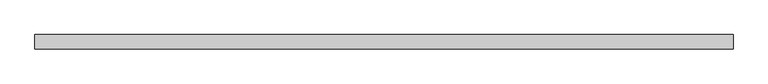
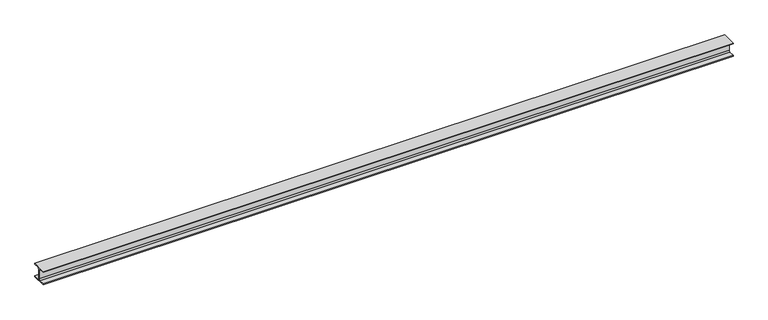
"""IFC4 building model written with IfcOpenShell, lengths in millimetres: beam geometry, NLRS_28_SF_LIB_stalen ligger HEB-AV-CWV-MMBS-SRP_gen_rsf : stalen ligger_gen__HEB 260."""

from ifc_helpers import new_model, si_unit, point, frame, frame_2d, origin, place, context, project, spatial, polyline, circle_curve, trimmed, segment, composite_curve, outline, extrude, source, transform, mapped, element, save


def beam_3eaeb734(model_context):
    return source(origin(), model_context, "Body", "SweptSolid", [
        extrude(outline(composite_curve([segment(polyline([(-130.0, 112.5), (-130.0, 130.0), (130.0, 130.0), (130.0, 112.5), (29.0, 112.5)]), True, "CONTINUOUS"), segment(trimmed(circle_curve(frame_2d((29.0, 88.5)), 24.0), [point((29.0, 112.5))], [point((5.0, 88.5))], True, "CARTESIAN"), True, "CONTINUOUS"), segment(polyline([(5.0, 88.5), (5.0, -88.5)]), True, "CONTINUOUS"), segment(trimmed(circle_curve(frame_2d((29.0, -88.5)), 24.0), [point((5.0, -88.5))], [point((29.0, -112.5))], True, "CARTESIAN"), True, "CONTINUOUS"), segment(polyline([(29.0, -112.5), (130.0, -112.5), (130.0, -130.0), (-130.0, -130.0), (-130.0, -112.5), (-29.0, -112.5)]), True, "CONTINUOUS"), segment(trimmed(circle_curve(frame_2d((-29.0, -88.5)), 24.0), [point((-29.0, -112.5))], [point((-5.0, -88.5))], True, "CARTESIAN"), True, "CONTINUOUS"), segment(polyline([(-5.0, -88.5), (-5.0, 88.5)]), True, "CONTINUOUS"), segment(trimmed(circle_curve(frame_2d((-29.0, 88.5)), 24.0), [point((-5.0, 88.5))], [point((-29.0, 112.5))], True, "CARTESIAN"), True, "CONTINUOUS"), segment(polyline([(-29.0, 112.5), (-130.0, 112.5)]), True, "CONTINUOUS")], self_intersect=False)), frame((-6349.0, 0.0, 0.0), z_axis=(1.0, 0.0, 0.0), x_axis=(0.0, 1.0, 0.0)), (0.0, 0.0, 1.0), 12698.0),
    ])


if __name__ == "__main__":
    model = new_model("IFC4")
    model_context = context("Model", 3, world=origin())
    ifc_project = project(units=[si_unit("LENGTHUNIT", "METRE", prefix="MILLI")], contexts=[model_context])
    site = spatial("IfcSite", under=ifc_project)
    building = spatial("IfcBuilding", under=site)
    placement = place(None, origin())
    beam_shape = beam_3eaeb734(model_context)
    element("IfcBeam", 1, ObjectType="NLRS_28_SF_LIB_stalen ligger HEB-AV-CWV-MMBS-SRP_gen_rsf : stalen ligger_gen__HEB 260", at=placement, inside=building, context=model_context, shape_type="MappedRepresentation", body=[
        mapped(beam_shape, transform((0.0, 0.0, 0.0), x_axis=(1.0, 0.0, 0.0), y_axis=(0.0, 1.0, 0.0), z_axis=(0.0, 0.0, 1.0))),
    ])
    save(model, "model.ifc")

# Revit data of these elements
# Type "NLRS_28_SF_LIB_stalen ligger HEB-AV-CWV-MMBS-SRP_gen_rsf : stalen ligger_gen__HEB 260"
#   Type IfcGUID = "0zo1UjqZ91lRsfCKsOOa5a"
#   IfcExportAs = "IfcBeamType"
#   Type Comments = "HEB260"
#   Model = " "
#   Manufacturer = " "
#   Fire Rating = " "
#   Description = "stalen ligger HEB260"
#   Assembly Code = "28.11"
#   ra = 24 mm
#   vz = 130 mm
#   vy = 130 mm
#   vpz = 130 mm
#   vpy = 130 mm
#   NLRS_C_lengte [instance default] = 1500 mm
#   Length [instance default] = 1500 mm
#   bf = 260 mm
#   d = 260 mm
#   tf = 17.5 mm
#   tw = 10 mm
#   Structural Material = NLRS_h2_staal_gen_rsf
#   Keynote = ""
# Element 1 (IfcBeam, "NLRS_28_SF_LIB_stalen ligger HEB-AV-CWV-MMBS-SRP_gen_rsf : stalen ligger_gen__HEB 260")
#   NLRS_C_lengte = 12698 mm
#   Materials on its faces: "NLRS_h2_staal_gen_rsf"
# Materials
#   "NLRS_h2_staal_gen_rsf": class "H - Metaal", colour RGB 189 187 185, transparency 0, Keynote = "h2", Manufacturer = "Revit Standards Foundation", URL = "www.revitstandards.org", Description = "staal", Cost = 0
